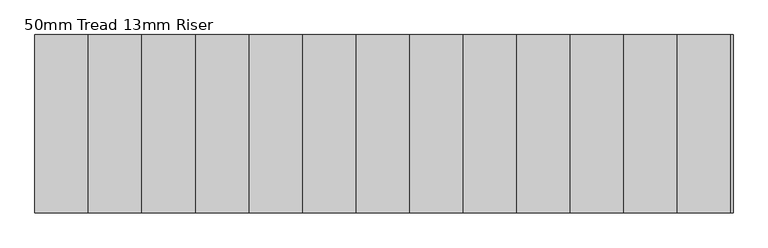
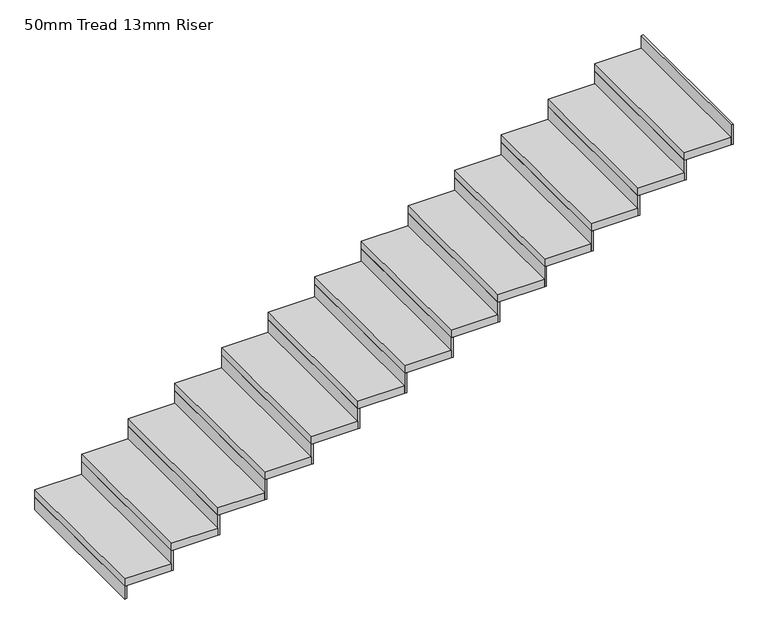
"""IFC4 building model written with IfcOpenShell, lengths in millimetres: stair flight geometry, 50mm Tread 13mm Riser."""

from ifc_helpers import new_model, si_unit, frame, origin, origin_with_axes, place, context, project, spatial, polyline, outline, extrude, source, transform, mapped, element, save


def stair_flight_50mm_tread_13mm_riser_7b17f1ba(model_context):
    return source(origin(), model_context, "Body", "SweptSolid", [
        extrude(outline(polyline([(17662.336337, -3576.2808257), (17649.836337, -3576.2808257), (17649.836337, -2576.2808257), (17662.336337, -2576.2808257), (17662.336337, -3576.2808257)])), origin_with_axes(), (0.0, 0.0, 1.0), 86.3636364),
        extrude(outline(polyline([(17949.836337, -2576.2808257), (17949.836337, -3576.2808257), (17649.836337, -3576.2808257), (17649.836337, -2576.2808257), (17949.836337, -2576.2808257)])), frame((0.0, 0.0, 86.3636364), z_axis=(0.0, 0.0, 1.0), x_axis=(1.0, 0.0, 0.0)), (0.0, 0.0, 1.0), 50.0),
        extrude(outline(polyline([(17962.336337, -3576.2808257), (17949.836337, -3576.2808257), (17949.836337, -2576.2808257), (17962.336337, -2576.2808257), (17962.336337, -3576.2808257)])), frame((0.0, 0.0, 86.3636364), z_axis=(0.0, 0.0, 1.0), x_axis=(1.0, 0.0, 0.0)), (0.0, 0.0, 1.0), 136.3636364),
        extrude(outline(polyline([(18249.836337, -2576.2808257), (18249.836337, -3576.2808257), (17949.836337, -3576.2808257), (17949.836337, -2576.2808257), (18249.836337, -2576.2808257)])), frame((0.0, 0.0, 222.7272727), z_axis=(0.0, 0.0, 1.0), x_axis=(1.0, 0.0, 0.0)), (0.0, 0.0, 1.0), 50.0),
        extrude(outline(polyline([(18262.336337, -3576.2808257), (18249.836337, -3576.2808257), (18249.836337, -2576.2808257), (18262.336337, -2576.2808257), (18262.336337, -3576.2808257)])), frame((0.0, 0.0, 222.7272727), z_axis=(0.0, 0.0, 1.0), x_axis=(1.0, 0.0, 0.0)), (0.0, 0.0, 1.0), 136.3636364),
        extrude(outline(polyline([(18549.836337, -2576.2808257), (18549.836337, -3576.2808257), (18249.836337, -3576.2808257), (18249.836337, -2576.2808257), (18549.836337, -2576.2808257)])), frame((0.0, 0.0, 359.0909091), z_axis=(0.0, 0.0, 1.0), x_axis=(1.0, 0.0, 0.0)), (0.0, 0.0, 1.0), 50.0),
        extrude(outline(polyline([(18562.336337, -3576.2808257), (18549.836337, -3576.2808257), (18549.836337, -2576.2808257), (18562.336337, -2576.2808257), (18562.336337, -3576.2808257)])), frame((0.0, 0.0, 359.0909091), z_axis=(0.0, 0.0, 1.0), x_axis=(1.0, 0.0, 0.0)), (0.0, 0.0, 1.0), 136.3636364),
        extrude(outline(polyline([(18849.836337, -2576.2808257), (18849.836337, -3576.2808257), (18549.836337, -3576.2808257), (18549.836337, -2576.2808257), (18849.836337, -2576.2808257)])), frame((0.0, 0.0, 495.4545455), z_axis=(0.0, 0.0, 1.0), x_axis=(1.0, 0.0, 0.0)), (0.0, 0.0, 1.0), 50.0),
        extrude(outline(polyline([(18862.336337, -3576.2808257), (18849.836337, -3576.2808257), (18849.836337, -2576.2808257), (18862.336337, -2576.2808257), (18862.336337, -3576.2808257)])), frame((0.0, 0.0, 495.4545455), z_axis=(0.0, 0.0, 1.0), x_axis=(1.0, 0.0, 0.0)), (0.0, 0.0, 1.0), 136.3636364),
        extrude(outline(polyline([(19149.836337, -2576.2808257), (19149.836337, -3576.2808257), (18849.836337, -3576.2808257), (18849.836337, -2576.2808257), (19149.836337, -2576.2808257)])), frame((0.0, 0.0, 631.8181818), z_axis=(0.0, 0.0, 1.0), x_axis=(1.0, 0.0, 0.0)), (0.0, 0.0, 1.0), 50.0),
        extrude(outline(polyline([(19162.336337, -3576.2808257), (19149.836337, -3576.2808257), (19149.836337, -2576.2808257), (19162.336337, -2576.2808257), (19162.336337, -3576.2808257)])), frame((0.0, 0.0, 631.8181818), z_axis=(0.0, 0.0, 1.0), x_axis=(1.0, 0.0, 0.0)), (0.0, 0.0, 1.0), 136.3636364),
        extrude(outline(polyline([(19449.836337, -2576.2808257), (19449.836337, -3576.2808257), (19149.836337, -3576.2808257), (19149.836337, -2576.2808257), (19449.836337, -2576.2808257)])), frame((0.0, 0.0, 768.1818182), z_axis=(0.0, 0.0, 1.0), x_axis=(1.0, 0.0, 0.0)), (0.0, 0.0, 1.0), 50.0),
        extrude(outline(polyline([(19462.336337, -3576.2808257), (19449.836337, -3576.2808257), (19449.836337, -2576.2808257), (19462.336337, -2576.2808257), (19462.336337, -3576.2808257)])), frame((0.0, 0.0, 768.1818182), z_axis=(0.0, 0.0, 1.0), x_axis=(1.0, 0.0, 0.0)), (0.0, 0.0, 1.0), 136.3636364),
        extrude(outline(polyline([(19749.836337, -2576.2808257), (19749.836337, -3576.2808257), (19449.836337, -3576.2808257), (19449.836337, -2576.2808257), (19749.836337, -2576.2808257)])), frame((0.0, 0.0, 904.5454545), z_axis=(0.0, 0.0, 1.0), x_axis=(1.0, 0.0, 0.0)), (0.0, 0.0, 1.0), 50.0),
        extrude(outline(polyline([(19762.336337, -3576.2808257), (19749.836337, -3576.2808257), (19749.836337, -2576.2808257), (19762.336337, -2576.2808257), (19762.336337, -3576.2808257)])), frame((0.0, 0.0, 904.5454545), z_axis=(0.0, 0.0, 1.0), x_axis=(1.0, 0.0, 0.0)), (0.0, 0.0, 1.0), 136.3636364),
        extrude(outline(polyline([(20049.836337, -2576.2808257), (20049.836337, -3576.2808257), (19749.836337, -3576.2808257), (19749.836337, -2576.2808257), (20049.836337, -2576.2808257)])), frame((0.0, 0.0, 1040.9090909), z_axis=(0.0, 0.0, 1.0), x_axis=(1.0, 0.0, 0.0)), (0.0, 0.0, 1.0), 50.0),
        extrude(outline(polyline([(20062.336337, -3576.2808257), (20049.836337, -3576.2808257), (20049.836337, -2576.2808257), (20062.336337, -2576.2808257), (20062.336337, -3576.2808257)])), frame((0.0, 0.0, 1040.9090909), z_axis=(0.0, 0.0, 1.0), x_axis=(1.0, 0.0, 0.0)), (0.0, 0.0, 1.0), 136.3636364),
        extrude(outline(polyline([(20349.836337, -2576.2808257), (20349.836337, -3576.2808257), (20049.836337, -3576.2808257), (20049.836337, -2576.2808257), (20349.836337, -2576.2808257)])), frame((0.0, 0.0, 1177.2727273), z_axis=(0.0, 0.0, 1.0), x_axis=(1.0, 0.0, 0.0)), (0.0, 0.0, 1.0), 50.0),
        extrude(outline(polyline([(20362.336337, -3576.2808257), (20349.836337, -3576.2808257), (20349.836337, -2576.2808257), (20362.336337, -2576.2808257), (20362.336337, -3576.2808257)])), frame((0.0, 0.0, 1177.2727273), z_axis=(0.0, 0.0, 1.0), x_axis=(1.0, 0.0, 0.0)), (0.0, 0.0, 1.0), 136.3636364),
        extrude(outline(polyline([(20649.836337, -2576.2808257), (20649.836337, -3576.2808257), (20349.836337, -3576.2808257), (20349.836337, -2576.2808257), (20649.836337, -2576.2808257)])), frame((0.0, 0.0, 1313.6363636), z_axis=(0.0, 0.0, 1.0), x_axis=(1.0, 0.0, 0.0)), (0.0, 0.0, 1.0), 50.0),
        extrude(outline(polyline([(20662.336337, -3576.2808257), (20649.836337, -3576.2808257), (20649.836337, -2576.2808257), (20662.336337, -2576.2808257), (20662.336337, -3576.2808257)])), frame((0.0, 0.0, 1313.6363636), z_axis=(0.0, 0.0, 1.0), x_axis=(1.0, 0.0, 0.0)), (0.0, 0.0, 1.0), 136.3636364),
        extrude(outline(polyline([(20949.836337, -2576.2808257), (20949.836337, -3576.2808257), (20649.836337, -3576.2808257), (20649.836337, -2576.2808257), (20949.836337, -2576.2808257)])), frame((0.0, 0.0, 1450.0), z_axis=(0.0, 0.0, 1.0), x_axis=(1.0, 0.0, 0.0)), (0.0, 0.0, 1.0), 50.0),
        extrude(outline(polyline([(20962.336337, -3576.2808257), (20949.836337, -3576.2808257), (20949.836337, -2576.2808257), (20962.336337, -2576.2808257), (20962.336337, -3576.2808257)])), frame((0.0, 0.0, 1450.0), z_axis=(0.0, 0.0, 1.0), x_axis=(1.0, 0.0, 0.0)), (0.0, 0.0, 1.0), 136.3636364),
        extrude(outline(polyline([(21249.836337, -2576.2808257), (21249.836337, -3576.2808257), (20949.836337, -3576.2808257), (20949.836337, -2576.2808257), (21249.836337, -2576.2808257)])), frame((0.0, 0.0, 1586.3636364), z_axis=(0.0, 0.0, 1.0), x_axis=(1.0, 0.0, 0.0)), (0.0, 0.0, 1.0), 50.0),
        extrude(outline(polyline([(21262.336337, -3576.2808257), (21249.836337, -3576.2808257), (21249.836337, -2576.2808257), (21262.336337, -2576.2808257), (21262.336337, -3576.2808257)])), frame((0.0, 0.0, 1586.3636364), z_axis=(0.0, 0.0, 1.0), x_axis=(1.0, 0.0, 0.0)), (0.0, 0.0, 1.0), 136.3636364),
        extrude(outline(polyline([(21562.336337, -3576.2808257), (21549.836337, -3576.2808257), (21549.836337, -2576.2808257), (21562.336337, -2576.2808257), (21562.336337, -3576.2808257)])), frame((0.0, 0.0, 1722.7272727), z_axis=(0.0, 0.0, 1.0), x_axis=(1.0, 0.0, 0.0)), (0.0, 0.0, 1.0), 136.3636364),
        extrude(outline(polyline([(21549.836337, -2576.2808257), (21549.836337, -3576.2808257), (21249.836337, -3576.2808257), (21249.836337, -2576.2808257), (21549.836337, -2576.2808257)])), frame((0.0, 0.0, 1722.7272727), z_axis=(0.0, 0.0, 1.0), x_axis=(1.0, 0.0, 0.0)), (0.0, 0.0, 1.0), 50.0),
    ])


if __name__ == "__main__":
    model = new_model("IFC4")
    model_context = context("Model", 3, world=origin())
    ifc_project = project(units=[si_unit("LENGTHUNIT", "METRE", prefix="MILLI")], contexts=[model_context])
    site = spatial("IfcSite", under=ifc_project)
    building = spatial("IfcBuilding", under=site)
    placement = place(None, origin())
    stair_flight_50mm_tread_13mm_riser_shape = stair_flight_50mm_tread_13mm_riser_7b17f1ba(model_context)
    element("IfcStairFlight", 1, ObjectType="50mm Tread 13mm Riser", at=placement, inside=building, context=model_context, shape_type="MappedRepresentation", body=[
        mapped(stair_flight_50mm_tread_13mm_riser_shape, transform((0.0, 0.0, 0.0), x_axis=(1.0, 0.0, 0.0), y_axis=(0.0, 1.0, 0.0), z_axis=(0.0, 0.0, 1.0))),
    ])
    save(model, "model.ifc")
